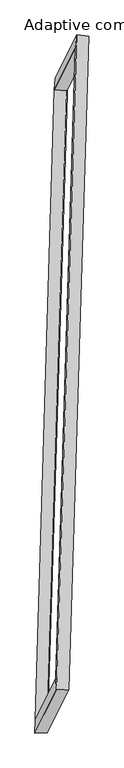
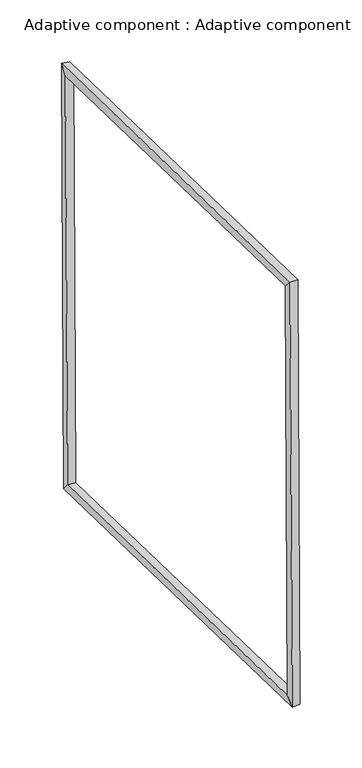
"""IFC4 building model written with IfcOpenShell, lengths in millimetres: proxy geometry, Adaptive component : Adaptive component."""

from ifc_helpers import new_model, si_unit, origin, place, context, project, spatial, faceted_brep, source, transform, mapped, element, save


def adaptive_component_adaptive_component_2f7eb678(model_context):
    return source(origin(), model_context, "Body", "Brep", [
        faceted_brep([(81.101095, 1333.7223956, 2921.4220665), (145.7296192, 1327.9347251, 2916.2715375), (44.3173672, -1954.4712313, 3130.7080033), (-20.5235032, -1955.5565618, 3136.3075391), (88.6155286, 1402.514608, 2981.8314499), (-17.0094328, -2016.2439283, 3205.1757004), (153.2440527, 1396.7269374, 2976.6809208), (47.8314376, -2015.1585978, 3199.5761647), (-63.1673355, -2170.5363525, -227.4601311), (-128.228196, -2172.063906, -228.7337959), (-128.8584915, -2241.0822527, -289.3489699), (-63.797631, -2239.5546993, -288.0753052), (38.2449166, 1111.8696039, -441.896597), (-26.6035977, 1117.2150515, -443.6192684), (-23.2335302, 1177.6762835, -512.6932205), (41.6149841, 1172.3308359, -510.9705491)], [[[0, 1, 2, 3]], [[4, 0, 3, 5]], [[6, 4, 5, 7]], [[1, 6, 7, 2]], [[3, 2, 8, 9]], [[5, 3, 9, 10]], [[7, 5, 10, 11]], [[2, 7, 11, 8]], [[9, 8, 12, 13]], [[10, 9, 13, 14]], [[11, 10, 14, 15]], [[8, 11, 15, 12]], [[13, 12, 1, 0]], [[14, 13, 0, 4]], [[15, 14, 4, 6]], [[12, 15, 6, 1]]]),
    ])


if __name__ == "__main__":
    model = new_model("IFC4")
    model_context = context("Model", 3, world=origin())
    ifc_project = project(units=[si_unit("LENGTHUNIT", "METRE", prefix="MILLI")], contexts=[model_context])
    site = spatial("IfcSite", under=ifc_project)
    building = spatial("IfcBuilding", under=site)
    placement = place(None, origin())
    adaptive_component_adaptive_component_shape = adaptive_component_adaptive_component_2f7eb678(model_context)
    element("IfcBuildingElementProxy", 1, Name="Adaptive component : Adaptive component", ObjectType="Adaptive component : Adaptive component", at=placement, inside=building, context=model_context, shape_type="MappedRepresentation", body=[
        mapped(adaptive_component_adaptive_component_shape, transform((0.0, 0.0, 0.0), x_axis=(1.0, 0.0, 0.0), y_axis=(0.0, 1.0, 0.0), z_axis=(0.0, 0.0, 1.0))),
    ])
    save(model, "model.ifc")

# Revit data of these elements
# Type "Adaptive component : Adaptive component"
#   r [instance default] = 2063.125 mm
#   2r [instance default] = 4126.251 mm
#   Number [instance default] = 5
#   Default Elevation = 0
# Element 1 (IfcBuildingElementProxy, "Adaptive component : Adaptive component")
#   r = 2448.199 mm
#   2r = 4896.399 mm
#   Number = 19
